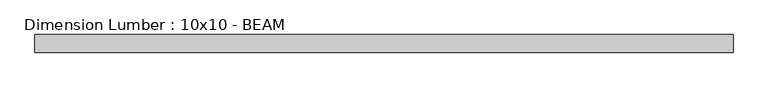
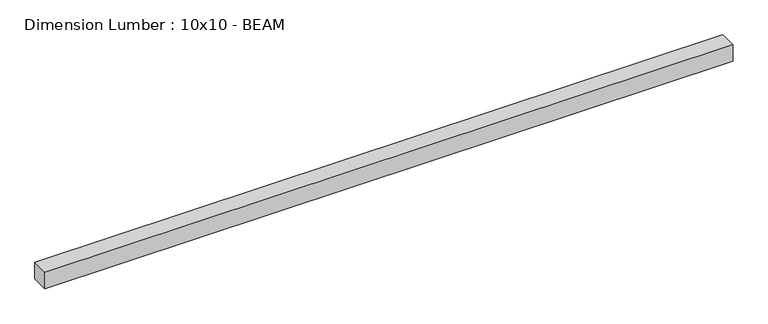
"""IFC4 building model written with IfcOpenShell, lengths in millimetres: beam geometry, Dimension Lumber : 10x10 - BEAM."""

from ifc_helpers import new_model, si_unit, frame, origin, place, context, project, spatial, polyline, outline, extrude, source, transform, mapped, element, save


def dimension_lumber_10x10_beam_82f4ea42(model_context):
    return source(origin(), model_context, "Body", "SweptSolid", [
        extrude(outline(polyline([(4648.2, 117.475), (4648.2, -117.475), (-4648.2, -117.475), (-4648.2, 117.475), (4648.2, 117.475)])), frame((0.0, 0.0, -117.475), z_axis=(0.0, 0.0, 1.0), x_axis=(1.0, 0.0, 0.0)), (0.0, 0.0, 1.0), 234.95),
    ])


if __name__ == "__main__":
    model = new_model("IFC4")
    model_context = context("Model", 3, world=origin())
    ifc_project = project(units=[si_unit("LENGTHUNIT", "METRE", prefix="MILLI")], contexts=[model_context])
    site = spatial("IfcSite", under=ifc_project)
    building = spatial("IfcBuilding", under=site)
    placement = place(None, origin())
    dimension_lumber_10x10_beam_shape = dimension_lumber_10x10_beam_82f4ea42(model_context)
    element("IfcBeam", 1, ObjectType="Dimension Lumber : 10x10 - BEAM", at=placement, inside=building, context=model_context, shape_type="MappedRepresentation", body=[
        mapped(dimension_lumber_10x10_beam_shape, transform((0.0, 0.0, 0.0), x_axis=(1.0, 0.0, 0.0), y_axis=(0.0, 1.0, 0.0), z_axis=(0.0, 0.0, 1.0))),
    ])
    save(model, "model.ifc")

# Revit data of these elements
# Type "Dimension Lumber : 10x10 - BEAM"
#   Assembly Code = "B10"
#   A = 0.0755556 SF
#   Length [instance default] = 5' - 0"
#   b = 0' - 9 1/4"
#   d = 0' - 9 1/4"
#   Structural Material = (4) CHARRED SISTERED 2X10s AT BEAM
# Element 1 (IfcBeam, "Dimension Lumber : 10x10 - BEAM")
#   Materials on its faces: "(4) CHARRED SISTERED 2X10s AT BEAM"
# Materials
#   "(4) CHARRED SISTERED 2X10s AT BEAM": class "Wood", colour RGB 144 144 144, transparency 0, Description = "Pinus Echinata", Cost = 0
